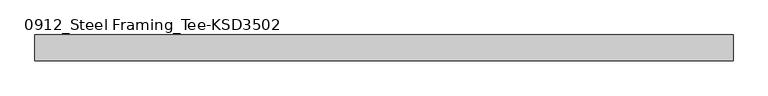
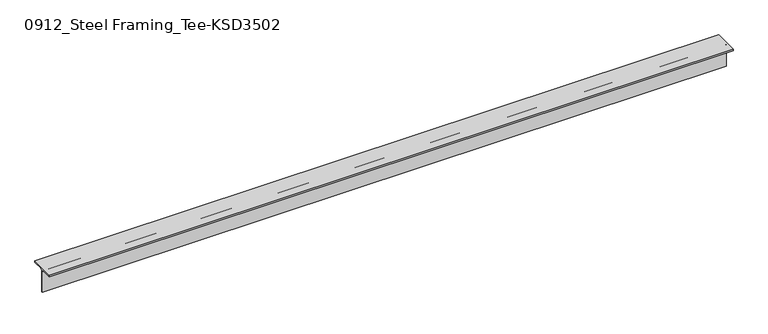
"""IFC4 building model written with IfcOpenShell, lengths in millimetres: member geometry, 0912_Steel Framing_Tee-KSD3502 : H_SB_ASB_CT-150x150x6.5x9."""

from ifc_helpers import new_model, si_unit, point, frame, frame_2d, origin, place, context, project, spatial, polyline, circle_curve, trimmed, segment, composite_curve, outline, extrude, source, transform, mapped, element, save


def member_0912_steel_framing_tee_ksd3502_5e97d94b(model_context):
    return source(origin(), model_context, "Body", "SweptSolid", [
        extrude(outline(composite_curve([segment(polyline([(-75.0, 75.0), (75.0, 75.0), (75.0, 66.0), (16.25, 66.0)]), True, "CONTINUOUS"), segment(trimmed(circle_curve(frame_2d((16.25, 53.0)), 13.0), [point((16.25, 66.0))], [point((3.25, 53.0))], True, "CARTESIAN"), True, "CONTINUOUS"), segment(polyline([(3.25, 53.0), (3.25, -75.0), (-3.25, -75.0), (-3.25, 53.0)]), True, "CONTINUOUS"), segment(trimmed(circle_curve(frame_2d((-16.25, 53.0)), 13.0), [point((-3.25, 53.0))], [point((-16.25, 66.0))], True, "CARTESIAN"), True, "CONTINUOUS"), segment(polyline([(-16.25, 66.0), (-75.0, 66.0), (-75.0, 75.0)]), True, "CONTINUOUS")], self_intersect=False)), frame((-2046.1, 0.0, 0.0), z_axis=(1.0, 0.0, 0.0), x_axis=(0.0, 1.0, 0.0)), (0.0, 0.0, 1.0), 4074.9),
    ])


if __name__ == "__main__":
    model = new_model("IFC4")
    model_context = context("Model", 3, world=origin())
    ifc_project = project(units=[si_unit("LENGTHUNIT", "METRE", prefix="MILLI")], contexts=[model_context])
    site = spatial("IfcSite", under=ifc_project)
    building = spatial("IfcBuilding", under=site)
    placement = place(None, origin())
    member_0912_steel_framing_tee_ksd3502_shape = member_0912_steel_framing_tee_ksd3502_5e97d94b(model_context)
    element("IfcMember", 1, ObjectType="0912_Steel Framing_Tee-KSD3502 : H_SB_ASB_CT-150x150x6.5x9", at=placement, inside=building, context=model_context, shape_type="MappedRepresentation", body=[
        mapped(member_0912_steel_framing_tee_ksd3502_shape, transform((0.0, 0.0, 0.0), x_axis=(1.0, 0.0, 0.0), y_axis=(0.0, 1.0, 0.0), z_axis=(0.0, 0.0, 1.0))),
    ])
    save(model, "model.ifc")

# Revit data of these elements
# Type "0912_Steel Framing_Tee-KSD3502 : H_SB_ASB_CT-150x150x6.5x9"
#   H_WM Code_1 = "S01AA003-00001 | Main Steel Structure Fabrication Work | Shelter/Building | Light Steel - Standard (30KG/M>Weight) | Material: (   )"
#   H_WM Code_2 = "S03AA029-00001 | Main Steel Structure Erection Work | Shelter/Building | Light Steel (30KG/M>Weight) | Material: (   )"
#   H_WM Code_3 = "S01AA010-00001 | Main Steel Structure Fabrication Work | Shelter/Building | Steel Painting/Coating | for Non-Fireproofed Steel Surface, Surface Preparation, Primer, Second & Final Coat | Material: (   )"
#   H_Q'ty Cal Type Tag = "SB-Q2"
#   Width = 15.0 cm
#   Web Thickness = 0.65 cm
#   Web Fillet = 1.3 cm
#   Section Area = 23.39 cm²
#   Perimeter = 0.60 m²/m
#   Nominal Weight = 18.40 kgf/m
#   Height = 15.0 cm
#   Flange Thickness = 0.9 cm
#   Centroid Vertical = 7.5 cm
#   Centroid Horizontal = 7.5 cm
#   Length [instance default] = 1.5000 m
#   Structural Material [instance default] = Steel, 45-345
#   Warping Constant = (empty or 0)
#   Torsional Moment of Inertia = 0
#   Section Name Key = ""
#   Plastic Modulus weak axis = 0
#   Plastic Modulus strong axis = 0
#   Moment of Inertia weak axis = 0
#   Moment of Inertia strong axis = 0
#   Elastic Modulus weak axis = 0
#   Elastic Modulus strong axis = 0
#   Bolt Spacing = 0
#   Assembly Code = ""
# Element 1 (IfcMember, "0912_Steel Framing_Tee-KSD3502 : H_SB_ASB_CT-150x150x6.5x9")
#   Structural Material = none
# Materials
#   "Steel, 45-345": class "Metal", colour RGB 189 187 185, transparency 0, Description = "Steel 345 MPa", Cost = 0
